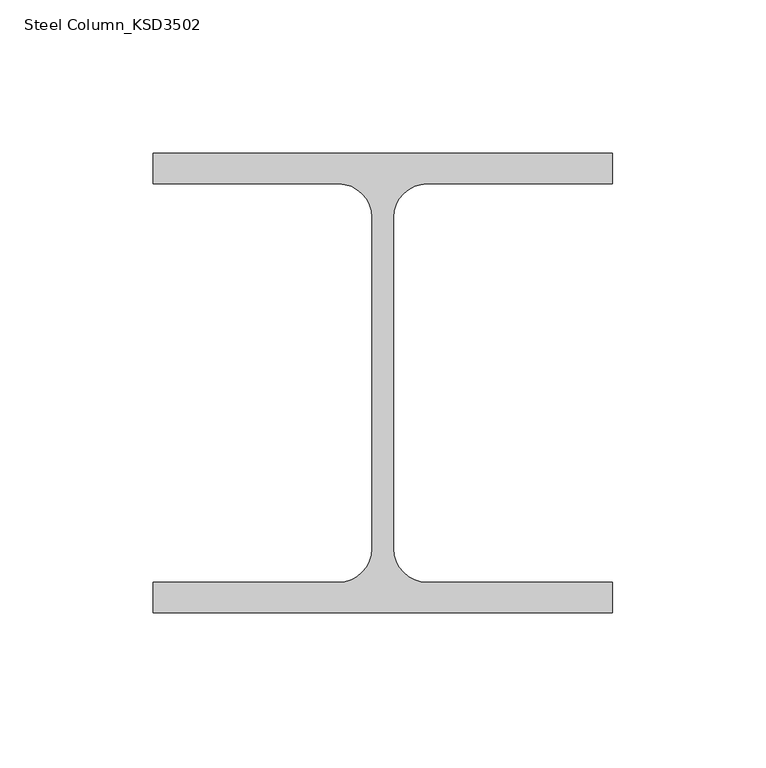
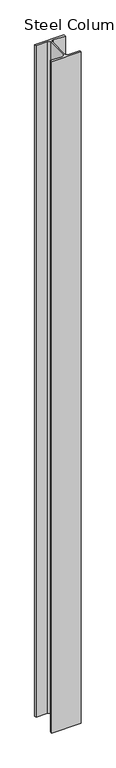
"""IFC4 building model written with IfcOpenShell, lengths in millimetres: column geometry, Steel Column_KSD3502 : H_SC_ASC_H-150×150x7x10."""

from ifc_helpers import new_model, si_unit, point, frame, frame_2d, origin, place, context, project, spatial, polyline, circle_curve, trimmed, segment, composite_curve, outline, extrude, source, transform, mapped, element, save


def steel_column_ksd3502_0d026061(model_context):
    return source(origin(), model_context, "Body", "SweptSolid", [
        extrude(outline(composite_curve([segment(polyline([(75.0, 75.0), (75.0, 65.0), (14.5, 65.0)]), True, "CONTINUOUS"), segment(trimmed(circle_curve(frame_2d((14.5, 54.0)), 11.0), [point((14.5, 65.0))], [point((3.5, 54.0))], True, "CARTESIAN"), True, "CONTINUOUS"), segment(polyline([(3.5, 54.0), (3.5, -54.0)]), True, "CONTINUOUS"), segment(trimmed(circle_curve(frame_2d((14.5, -54.0)), 11.0), [point((3.5, -54.0))], [point((14.5, -65.0))], True, "CARTESIAN"), True, "CONTINUOUS"), segment(polyline([(14.5, -65.0), (75.0, -65.0), (75.0, -75.0), (-75.0, -75.0), (-75.0, -65.0), (-14.5, -65.0)]), True, "CONTINUOUS"), segment(trimmed(circle_curve(frame_2d((-14.5, -54.0)), 11.0), [point((-14.5, -65.0))], [point((-3.5, -54.0))], True, "CARTESIAN"), True, "CONTINUOUS"), segment(polyline([(-3.5, -54.0), (-3.5, 54.0)]), True, "CONTINUOUS"), segment(trimmed(circle_curve(frame_2d((-14.5, 54.0)), 11.0), [point((-3.5, 54.0))], [point((-14.5, 65.0))], True, "CARTESIAN"), True, "CONTINUOUS"), segment(polyline([(-14.5, 65.0), (-75.0, 65.0), (-75.0, 75.0), (75.0, 75.0)]), True, "CONTINUOUS")], self_intersect=False)), frame((0.0, 0.0, 8299.9720055), z_axis=(0.0, 0.0, 1.0), x_axis=(1.0, 0.0, 0.0)), (0.0, 0.0, 1.0), 3610.0),
    ])


if __name__ == "__main__":
    model = new_model("IFC4")
    model_context = context("Model", 3, world=origin())
    ifc_project = project(units=[si_unit("LENGTHUNIT", "METRE", prefix="MILLI")], contexts=[model_context])
    site = spatial("IfcSite", under=ifc_project)
    building = spatial("IfcBuilding", under=site)
    placement = place(None, origin())
    steel_column_ksd3502_shape = steel_column_ksd3502_0d026061(model_context)
    element("IfcColumn", 1, ObjectType="Steel Column_KSD3502 : H_SC_ASC_H-150×150x7x10", at=placement, inside=building, context=model_context, shape_type="MappedRepresentation", body=[
        mapped(steel_column_ksd3502_shape, transform((0.0, 0.0, 0.0), x_axis=(1.0, 0.0, 0.0), y_axis=(0.0, 1.0, 0.0), z_axis=(0.0, 0.0, 1.0))),
    ])
    save(model, "model.ifc")

# Revit data of these elements
# Type "Steel Column_KSD3502 : H_SC_ASC_H-150×150x7x10"
#   Width = 15.0 cm
#   Web Thickness = 0.7 cm
#   Web Fillet = 1.1 cm
#   Warping Constant = 27562.5 cm⁶
#   Torsional Moment of Inertia = 11.6007 cm⁴
#   Section Area = 40.14 cm²
#   Plastic Modulus weak axis = 115.0 cm³
#   Plastic Modulus strong axis = 246.0 cm³
#   Perimeter = 1.27 m²/m
#   Nominal Weight = 31.50 kgf/m
#   Moment of Inertia weak axis = 563.00 cm⁴
#   Moment of Inertia strong axis = 1640.00 cm⁴
#   Height = 15.0 cm
#   Flange Thickness = 1.0 cm
#   Elastic Modulus weak axis = 75.1 cm³
#   Elastic Modulus strong axis = 219.0 cm³
#   Centroid Vertical = 7.5 cm
#   Centroid Horizontal = 7.5 cm
#   Bolt Spacing = 13.97 cm
#   Structural Material [instance default] = Steel, 45-345
#   Section Name Key = ""
#   Assembly Code = ""
# Element 1 (IfcColumn, "Steel Column_KSD3502 : H_SC_ASC_H-150×150x7x10")
#   Structural Material = none
# Materials
#   "Steel, 45-345": class "Metal", colour RGB 189 187 185, transparency 0, Description = "Steel 345 MPa", Cost = 0
